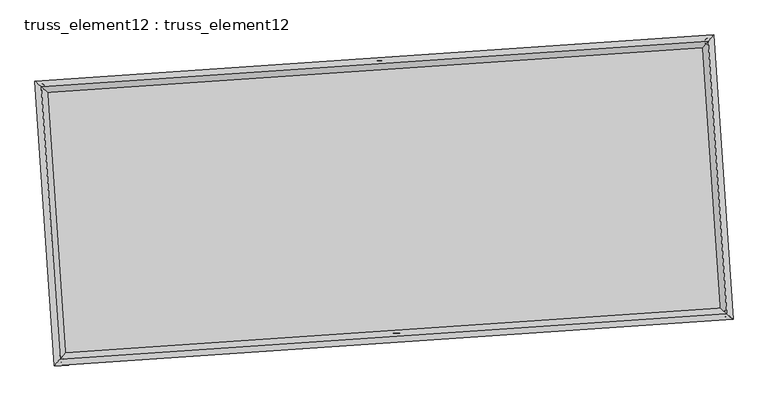
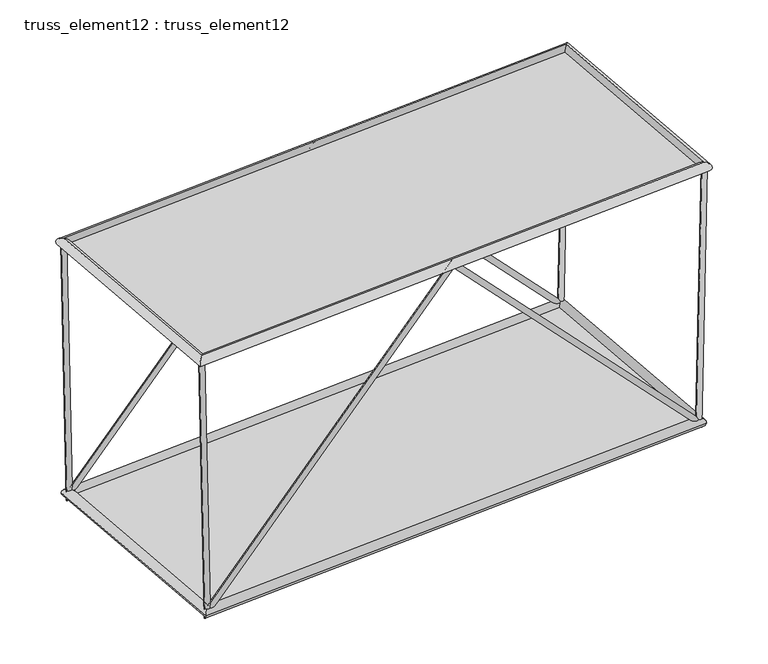
"""IFC4 building model written with IfcOpenShell, lengths in millimetres: plate geometry, truss_element12 : truss_element12."""

import ifcopenshell
import ifcopenshell.guid

model = None  # the IFC model being written
_history = None  # IfcOwnerHistory: only IFC2X3 demands one
_inside = {}  # id of a spatial element -> (the spatial element, [elements in it])
_under = {}  # id of a project, library or spatial element -> (it, [spatial elements below it])
_declared = {}  # id of a project -> (the project, [libraries it declares])
_typed = {}  # id of a type object -> (the type object, [elements of that type])
_made_of = {}  # id of a material, layer set ... -> (it, [elements and type objects made of it])


def new_model(schema):
    """Start an empty IFC model of exactly this schema.

    Asked for "IFC4X3", IfcOpenShell would pick the latest addendum, in which some entities
    have other attributes; the version numbers below select the first issue.
    IFC2X3 requires an IfcOwnerHistory on every rooted entity: one is made here for all.
    """
    global model, _history
    if schema == "IFC4X3":
        model = ifcopenshell.file(schema_version=(4, 3, 0, 0))
    else:
        model = ifcopenshell.file(schema=schema)
    _inside.clear()
    _under.clear()
    _declared.clear()
    _typed.clear()
    _made_of.clear()
    _history = None
    if model.schema == "IFC2X3":
        org = make("IfcOrganization", Name="unknown")
        user = make(
            "IfcPersonAndOrganization",
            ThePerson=make("IfcPerson", FamilyName="unknown"),
            TheOrganization=org,
        )
        app = make(
            "IfcApplication",
            ApplicationDeveloper=org,
            Version="unknown",
            ApplicationFullName="unknown",
            ApplicationIdentifier="unknown",
        )
        _history = make(
            "IfcOwnerHistory",
            OwningUser=user,
            OwningApplication=app,
            ChangeAction="ADDED",
            CreationDate=0,
        )
    return model


def make(cls, **values):
    """One entity of the class cls with the attributes given. An attribute that is None is left unset."""
    return model.create_entity(
        cls, **{name: value for name, value in values.items() if value is not None}
    )


def rooted(cls, **values):
    """An entity with a GlobalId (a new one), such as an element, a storey or a relation."""
    return make(cls, GlobalId=ifcopenshell.guid.new(), OwnerHistory=_history, **values)


def si_unit(unit_type, name, prefix=None):
    """IfcSIUnit, for example si_unit("LENGTHUNIT", "METRE", prefix="MILLI")."""
    return make("IfcSIUnit", UnitType=unit_type, Prefix=prefix, Name=name)


def assignment(units):
    """IfcUnitAssignment: the units of a project."""
    return None if units is None else make("IfcUnitAssignment", Units=units)


def point(xyz):
    """IfcCartesianPoint."""
    return None if xyz is None else make("IfcCartesianPoint", Coordinates=xyz)


def direction(xyz):
    """IfcDirection."""
    return None if xyz is None else make("IfcDirection", DirectionRatios=xyz)


def frame(location, z_axis=None, x_axis=None):
    """IfcAxis2Placement3D, a coordinate frame: its origin and axes. An axis left out is left unset."""
    return make(
        "IfcAxis2Placement3D",
        Location=point(location),
        Axis=direction(z_axis),
        RefDirection=direction(x_axis),
    )


def origin():
    """The frame at (0, 0, 0) with its axes left unset."""
    return frame((0.0, 0.0, 0.0))


def origin_with_axes():
    """The frame at (0, 0, 0) with the z axis (0, 0, 1) and the x axis (1, 0, 0) written out."""
    return frame((0.0, 0.0, 0.0), z_axis=(0.0, 0.0, 1.0), x_axis=(1.0, 0.0, 0.0))


def place(relative_to, where):
    """IfcLocalPlacement: puts the frame where relative to a parent placement (None: the world)."""
    return make(
        "IfcLocalPlacement", PlacementRelTo=relative_to, RelativePlacement=where
    )


def context(
    kind, dimensions, precision=None, world=None, true_north=None, identifier=None
):
    """IfcGeometricRepresentationContext, for example the 3D "Model" context."""
    return make(
        "IfcGeometricRepresentationContext",
        ContextIdentifier=identifier,
        ContextType=kind,
        CoordinateSpaceDimension=dimensions,
        Precision=precision,
        WorldCoordinateSystem=world,
        TrueNorth=true_north,
    )


def project(units=None, contexts=None):
    """IfcProject with its units and contexts."""
    return rooted(
        "IfcProject",
        Name="project",
        RepresentationContexts=contexts,
        UnitsInContext=assignment(units),
    )


def spatial(cls, under=None, at=None, **own):
    """A site, building, storey or space (cls), placed at a placement, below another one or the project."""
    s = rooted(cls, ObjectPlacement=at, **own)
    if under is not None:
        _under.setdefault(under.id(), (under, []))[1].append(s)
    return s


def polyline(points):
    """IfcPolyline through the points."""
    return make("IfcPolyline", Points=[point(p) for p in points])


def circle_curve(where, radius):
    """IfcCircle in the frame where."""
    return make("IfcCircle", Position=where, Radius=radius)


def ellipse_curve(where, semi_axis1, semi_axis2):
    """IfcEllipse in the frame where."""
    return make(
        "IfcEllipse", Position=where, SemiAxis1=semi_axis1, SemiAxis2=semi_axis2
    )


def outline(outer, holes=None, kind="AREA"):
    """IfcArbitraryClosedProfileDef: a profile drawn as a closed curve; with holes, ...WithVoids."""
    if holes is None:
        return make("IfcArbitraryClosedProfileDef", ProfileType=kind, OuterCurve=outer)
    return make(
        "IfcArbitraryProfileDefWithVoids",
        ProfileType=kind,
        OuterCurve=outer,
        InnerCurves=holes,
    )


def extrude(swept, where, along, depth):
    """IfcExtrudedAreaSolid: the profile swept, set in the frame where, extruded along a direction by depth."""
    return make(
        "IfcExtrudedAreaSolid",
        SweptArea=swept,
        Position=where,
        ExtrudedDirection=direction(along),
        Depth=depth,
    )


def shape(context_of_items, identifier, shape_type, items):
    """IfcShapeRepresentation: the items that make up one representation, for example the "Body"."""
    return make(
        "IfcShapeRepresentation",
        ContextOfItems=context_of_items,
        RepresentationIdentifier=identifier,
        RepresentationType=shape_type,
        Items=items,
    )


def source(mapping_origin, context_of_items, identifier, shape_type, items):
    """IfcRepresentationMap: a shape defined once, which mapped items show again and again."""
    return make(
        "IfcRepresentationMap",
        MappingOrigin=mapping_origin,
        MappedRepresentation=shape(context_of_items, identifier, shape_type, items),
    )


def transform(
    local_origin,
    x_axis=None,
    y_axis=None,
    z_axis=None,
    scale=None,
    scale2=None,
    scale3=None,
    uniform=True,
):
    """IfcCartesianTransformationOperator3D, or its non-uniform kind. x_axis, y_axis, z_axis: its Axis1, 2, 3."""
    if uniform:
        return make(
            "IfcCartesianTransformationOperator3D",
            Axis1=direction(x_axis),
            Axis2=direction(y_axis),
            LocalOrigin=point(local_origin),
            Scale=scale,
            Axis3=direction(z_axis),
        )
    return make(
        "IfcCartesianTransformationOperator3DnonUniform",
        Axis1=direction(x_axis),
        Axis2=direction(y_axis),
        LocalOrigin=point(local_origin),
        Scale=scale,
        Axis3=direction(z_axis),
        Scale2=scale2,
        Scale3=scale3,
    )


def mapped(mapping_source, mapping_target):
    """IfcMappedItem: shows the shape of a source again, moved by a transform."""
    return make(
        "IfcMappedItem", MappingSource=mapping_source, MappingTarget=mapping_target
    )


def made_of(thing, what):
    """Note that an element or type object is made of a material, layer set ...; save() writes the relation."""
    if what is not None:
        _made_of.setdefault(what.id(), (what, []))[1].append(thing)
    return thing


def element(
    cls,
    number,
    at=None,
    inside=None,
    cuts=None,
    type_object=None,
    material=None,
    context=None,
    identifier="Body",
    shape_type=None,
    held_by="IfcProductDefinitionShape",
    body=None,
    shapes=None,
    **own,
):
    """One element of the class cls, such as IfcWall. Its Tag is "e" and its number.

    at: its placement. inside: the storey or other place that contains it. cuts: it is an
    opening in that element (IfcRelVoidsElement). A single representation is given by context,
    identifier, shape_type and body (its items); several are given by shapes. held_by: the class
    of the entity that holds the representations. save() writes the other relations.
    """
    e = rooted(cls, Tag="e%d" % number, ObjectPlacement=at, **own)
    if body is not None:
        shapes = [shape(context, identifier, shape_type, body)]
    if shapes is not None:
        e.Representation = make(held_by, Representations=shapes)
    if inside is not None:
        _inside.setdefault(inside.id(), (inside, []))[1].append(e)
    if cuts is not None:
        rooted(
            "IfcRelVoidsElement", RelatingBuildingElement=cuts, RelatedOpeningElement=e
        )
    if type_object is not None:
        _typed.setdefault(type_object.id(), (type_object, []))[1].append(e)
    return made_of(e, material)


def aggregate(whole, parts):
    """IfcRelAggregates: a whole, such as a stair, and the parts it consists of."""
    return rooted("IfcRelAggregates", RelatingObject=whole, RelatedObjects=parts)


def save(model, path):
    """Write the relations noted so far, then the file.

    IfcRelAggregates (storeys below a building ...), IfcRelContainedInSpatialStructure (elements
    in a storey), IfcRelDefinesByType, IfcRelAssociatesMaterial and IfcRelDeclares: one each for
    every whole, place, type object, material and project.
    """
    for whole, parts in _under.values():
        aggregate(whole, parts)
    for where, things in _inside.values():
        rooted(
            "IfcRelContainedInSpatialStructure",
            RelatedElements=things,
            RelatingStructure=where,
        )
    for kind, things in _typed.values():
        rooted("IfcRelDefinesByType", RelatedObjects=things, RelatingType=kind)
    for what, things in _made_of.values():
        rooted("IfcRelAssociatesMaterial", RelatedObjects=things, RelatingMaterial=what)
    for by, libraries in _declared.values():
        rooted("IfcRelDeclares", RelatingContext=by, RelatedDefinitions=libraries)
    model.write(path)


def plane_surface(at):
    """IfcPlane: the flat surface through the origin of the frame at, square to its z axis."""
    return make("IfcPlane", Position=at)


def cylinder_surface(at, radius):
    """IfcCylindricalSurface: all points at the distance radius from the z axis of the frame at."""
    return make("IfcCylindricalSurface", Position=at, Radius=radius)


def advanced_brep(points, edges, surfaces, faces):
    """IfcAdvancedBrep: a solid bounded by faces that lie on surfaces and meet in shared edges.

    An edge is (start, end): straight between two places in points (the first is 0);
    or (start, end, curve); or (start, end, curve, False) where it runs against its curve.
    A face is (place in surfaces, loops), or (place, loops, False) where it looks against
    its surface's normal. A loop lists edges by number (the first is 1), with a minus sign
    where the edge is run from its end to its start. The first loop is the outer one.
    """
    corners = [point(p) for p in points]
    vertices = [make("IfcVertexPoint", VertexGeometry=c) for c in corners]
    made = []
    for start, end, *more in edges:
        made.append(
            make(
                "IfcEdgeCurve",
                EdgeStart=vertices[start],
                EdgeEnd=vertices[end],
                EdgeGeometry=more[0] if more else make("IfcPolyline", Points=[corners[start], corners[end]]),
                SameSense=more[1] if len(more) > 1 else True,
            )
        )
    hull = []
    for where, loops, *sense in faces:
        bounds = []
        for j, loop in enumerate(loops):
            ring = [make("IfcOrientedEdge", EdgeElement=made[abs(k) - 1], Orientation=k > 0) for k in loop]
            bounds.append(
                make(
                    "IfcFaceOuterBound" if j == 0 else "IfcFaceBound",
                    Bound=make("IfcEdgeLoop", EdgeList=ring),
                    Orientation=True,
                )
            )
        hull.append(make("IfcAdvancedFace", Bounds=bounds, FaceSurface=surfaces[where], SameSense=sense[0] if sense else True))
    return make("IfcAdvancedBrep", Outer=make("IfcClosedShell", CfsFaces=hull))


def truss_element12_truss_element12_abe7b1e7(model_context):
    return source(origin(), model_context, "Body", "SolidModel", [
        advanced_brep(
        [(-3770.8878019, 2268.9998903, 4999.9319376), (-3869.9687215, 2255.6402044, 4997.8129357), (-3667.5052192, 2276.0491556, 121.4949725), (-3761.4816636, 2263.0375245, -121.4949725), (1064.3047665, 2598.6932913, 5070.9753827), (1064.7442266, 2592.1195217, 4926.7446167), (5794.9719015, 2921.2595003, 121.4870027), (5889.7890755, 2921.1209882, -121.4870027), (5899.4888428, 2928.3861132, 4999.9186849), (5999.4656666, 2928.5994181, 4997.7764407)],
        [
            (0, 1, circle_curve(frame((-3820.4282617, 2262.3200473, 4998.8724366), z_axis=(-0.021186964059823055, -0.0014446585400489402, 0.9997744873298331), x_axis=(-0.1335973438749746, 0.9910347078393886, -0.0013991308907449146)), 50.0)),
            (1, 0, circle_curve(frame((-3820.4282617, 2262.3200473, 4998.8724366), z_axis=(-0.021186964059823055, -0.0014446585400489402, 0.9997744873298331), x_axis=(-0.1335973438749746, 0.9910347078393886, -0.0013991308907449146)), 50.0)),
            (0, 2),
            (2, 3, ellipse_curve(frame((-3714.4934414, 2269.54334, 0.0), z_axis=(-0.9296544314303254, -0.06338960173189395, 0.36293855749180226), x_axis=(0.36209777260493814, 0.02469007065143342, 0.9318130732533052)), 130.6694735, 50.0)),
            (3, 1),
            (3, 2, ellipse_curve(frame((-3714.4934414, 2269.54334, 0.0), z_axis=(-0.9296544314303254, -0.06338960173189395, 0.36293855749180226), x_axis=(0.36209777260493814, 0.02469007065143342, 0.9318130732533052)), 130.6694735, 50.0)),
            (2, 4),
            (4, 5, ellipse_curve(frame((1064.5244965, 2595.4064065, 4998.8599997), z_axis=(-0.9976833942347468, -0.06802823810322978, 6.073553142189921e-05), x_axis=(-6.0594831251560616e-05, -4.131731200348947e-06, -0.9999999981555977)), 72.2724119, 50.0)),
            (5, 3),
            (5, 4, ellipse_curve(frame((1064.5244965, 2595.4064065, 4998.8599997), z_axis=(-0.9976833942347468, -0.06802823810322978, 6.073553142189921e-05), x_axis=(-6.0594831251560616e-05, -4.131731200348947e-06, -0.9999999981555977)), 72.2724119, 50.0)),
            (4, 6),
            (6, 7, ellipse_curve(frame((5842.3804885, 2921.1902443, 0.0), z_axis=(-0.929718590145964, -0.06339397647082363, -0.3627734098362472), x_axis=(-0.36193300753109015, -0.024678835947378536, 0.9318773809443935)), 130.6518852, 50.0)),
            (7, 5),
            (7, 6, ellipse_curve(frame((5842.3804885, 2921.1902443, 0.0), z_axis=(-0.929718590145964, -0.06339397647082363, -0.3627734098362472), x_axis=(-0.36193300753109015, -0.024678835947378536, 0.9318773809443935)), 130.6518852, 50.0)),
            (8, 9, circle_curve(frame((5949.4772547, 2928.4927656, 4998.8475628), z_axis=(0.021419353246380234, 0.001460504275286309, 0.9997695125546532), x_axis=(-0.0021638448984886293, 0.999996658509091, -0.0014144772560226867)), 50.0)),
            (9, 8, circle_curve(frame((5949.4772547, 2928.4927656, 4998.8475628), z_axis=(0.021419353246380234, 0.001460504275286309, 0.9997695125546532), x_axis=(-0.0021638448984886293, 0.999996658509091, -0.0014144772560226867)), 50.0)),
            (6, 8),
            (9, 7),
        ],
        [
            plane_surface(frame((-3820.4282617, 2312.3199951, 4998.9446858), z_axis=(-0.021186964059822382, -0.0014446585400488944, 0.9997744873298331), x_axis=(0.9997755310838168, -3.061480063770717e-05, 0.021186941940879226))),
            cylinder_surface(frame((-3820.4282617, 2262.3200473, 4998.8724366), z_axis=(-0.021186964059823055, -0.0014446585400489402, 0.9997744873298331), x_axis=(-0.1335973438749746, 0.9910347078393886, -0.0013991308907449146)), 50.0),
            cylinder_surface(frame((-3714.4934414, 2269.54334, 0.0), z_axis=(-0.6902679812639986, -0.047066749688142194, -0.7220213536423408), x_axis=(-0.02042071364567827, 0.9987517920300755, -0.045583465981802296)), 50.0),
            cylinder_surface(frame((1064.5244965, 2595.4064065, 4998.8599997), z_axis=(-0.6901804746474645, -0.0470607829446048, 0.7221053905933964), x_axis=(-0.11534567202188306, 0.9922792199619508, -0.045577687277029266)), 50.0),
            plane_surface(frame((5949.4772547, 2878.492819, 4998.9206047), z_axis=(0.02141935324638098, 0.0014605042752824204, 0.9997695125546532), x_axis=(0.999770579336333, -3.129023561676551e-05, -0.021419330391363928))),
            cylinder_surface(frame((5842.3804885, 2921.1902443, 0.0), z_axis=(-0.021419353246380234, -0.001460504275286309, -0.9997695125546532), x_axis=(-0.0021638448984886293, 0.999996658509091, -0.0014144772560226867)), 50.0),
        ],
        [
            (0, [[1, 2]]),
            (1, [[-1, 3, 4, 5]]),
            (1, [[-2, -5, 6, -3]]),
            (2, [[-4, 7, 8, 9]]),
            (2, [[-6, -9, 10, -7]]),
            (3, [[-8, 11, 12, 13]]),
            (3, [[-10, -13, 14, -11]]),
            (4, [[15, 16]]),
            (5, [[-12, 17, -16, 18]]),
            (5, [[-14, -18, -15, -17]]),
        ],
    ),
        advanced_brep(
        [(-3498.774849, -1721.733694, 4999.9319376), (-3597.8557686, -1735.0933799, 4997.8129357), (-3395.3922663, -1714.6844287, 121.4949725), (-3489.3687107, -1727.6960598, -121.4949725), (1336.4177194, -1392.040293, 5070.9753827), (1336.8571795, -1398.6140626, 4926.7446167), (6067.0848544, -1069.474084, 121.4870027), (6161.9020284, -1069.6125961, -121.4870027), (6171.6017958, -1062.3474711, 4999.9186849), (6271.5786195, -1062.1341662, 4997.7764407)],
        [
            (0, 1, circle_curve(frame((-3548.3153088, -1728.413537, 4998.8724366), z_axis=(-0.021186964059823104, -0.001444658540048999, 0.9997744873298331), x_axis=(-0.13359734387497507, 0.9910347078393886, -0.0013991308907448728)), 50.0)),
            (1, 0, circle_curve(frame((-3548.3153088, -1728.413537, 4998.8724366), z_axis=(-0.021186964059823104, -0.001444658540048999, 0.9997744873298331), x_axis=(-0.13359734387497507, 0.9910347078393886, -0.0013991308907448728)), 50.0)),
            (0, 2),
            (2, 3, ellipse_curve(frame((-3442.3804885, -1721.1902443, 0.0), z_axis=(-0.9296544314303253, -0.06338960173189416, 0.36293855749180204), x_axis=(0.3620977726049378, 0.02469007065143343, 0.9318130732533053)), 130.6694735, 50.0)),
            (3, 1),
            (3, 2, ellipse_curve(frame((-3442.3804885, -1721.1902443, 0.0), z_axis=(-0.9296544314303253, -0.06338960173189416, 0.36293855749180204), x_axis=(0.3620977726049378, 0.02469007065143343, 0.9318130732533053)), 130.6694735, 50.0)),
            (2, 4),
            (4, 5, ellipse_curve(frame((1336.6374494, -1395.3271778, 4998.8599997), z_axis=(-0.9976833942347471, -0.06802823810322975, 6.073553142173877e-05), x_axis=(-6.059483125109933e-05, -4.1317312005027025e-06, -0.9999999981555977)), 72.2724119, 50.0)),
            (5, 3),
            (5, 4, ellipse_curve(frame((1336.6374494, -1395.3271778, 4998.8599997), z_axis=(-0.9976833942347471, -0.06802823810322975, 6.073553142173877e-05), x_axis=(-6.059483125109933e-05, -4.1317312005027025e-06, -0.9999999981555977)), 72.2724119, 50.0)),
            (4, 6),
            (6, 7, ellipse_curve(frame((6114.4934414, -1069.54334, 0.0), z_axis=(-0.929718590145964, -0.06339397647082334, -0.3627734098362472), x_axis=(-0.36193300753109015, -0.024678835947378446, 0.9318773809443935)), 130.6518852, 50.0)),
            (7, 5),
            (7, 6, ellipse_curve(frame((6114.4934414, -1069.54334, 0.0), z_axis=(-0.929718590145964, -0.06339397647082334, -0.3627734098362472), x_axis=(-0.36193300753109015, -0.024678835947378446, 0.9318773809443935)), 130.6518852, 50.0)),
            (8, 9, circle_curve(frame((6221.5902076, -1062.2408187, 4998.8475628), z_axis=(0.021419353246380123, 0.0014605042752862665, 0.9997695125546532), x_axis=(-0.0021638448984882684, 0.999996658509091, -0.001414477256022652)), 50.0)),
            (9, 8, circle_curve(frame((6221.5902076, -1062.2408187, 4998.8475628), z_axis=(0.021419353246380123, 0.0014605042752862665, 0.9997695125546532), x_axis=(-0.0021638448984882684, 0.999996658509091, -0.001414477256022652)), 50.0)),
            (6, 8),
            (9, 7),
        ],
        [
            plane_surface(frame((-3548.3153088, -1678.4135892, 4998.9446858), z_axis=(-0.021186964059822382, -0.001444658540048914, 0.9997744873298331), x_axis=(0.9997755310838168, -3.061480063770717e-05, 0.021186941940879226))),
            cylinder_surface(frame((-3548.3153088, -1728.413537, 4998.8724366), z_axis=(-0.021186964059823104, -0.001444658540048999, 0.9997744873298331), x_axis=(-0.13359734387497507, 0.9910347078393886, -0.0013991308907448728)), 50.0),
            cylinder_surface(frame((-3442.3804885, -1721.1902443, 0.0), z_axis=(-0.6902679812639982, -0.04706674968814228, -0.722021353642341), x_axis=(-0.020420713645678303, 0.9987517920300755, -0.04558346598180237)), 50.0),
            cylinder_surface(frame((1336.6374494, -1395.3271778, 4998.8599997), z_axis=(-0.6901804746474646, -0.04706078294460461, 0.7221053905933964), x_axis=(-0.11534567202188295, 0.9922792199619508, -0.04557768727702941)), 50.0),
            plane_surface(frame((6221.5902076, -1112.2407653, 4998.9206047), z_axis=(0.021419353246380984, 0.0014605042752824403, 0.9997695125546533), x_axis=(0.999770579336333, -3.129023561676551e-05, -0.021419330391363928))),
            cylinder_surface(frame((6114.4934414, -1069.54334, 0.0), z_axis=(-0.021419353246380123, -0.0014605042752862665, -0.9997695125546532), x_axis=(-0.0021638448984882684, 0.999996658509091, -0.001414477256022652)), 50.0),
        ],
        [
            (0, [[1, 2]]),
            (1, [[-1, 3, 4, 5]]),
            (1, [[-2, -5, 6, -3]]),
            (2, [[-4, 7, 8, 9]]),
            (2, [[-6, -9, 10, -7]]),
            (3, [[-8, 11, 12, 13]]),
            (3, [[-10, -13, 14, -11]]),
            (4, [[15, 16]]),
            (5, [[-12, 17, -16, 18]]),
            (5, [[-14, -18, -15, -17]]),
        ],
    ),
        advanced_brep(
        [(-3548.3217778, -1728.4207068, 4908.8724369), (-3548.3088398, -1728.4063671, 5088.8724364), (-3820.4208794, 2262.313822, 5088.8724364), (-3820.4356441, 2262.3262727, 4908.8724369), (5949.4712419, 2928.4856269, 5088.8475625), (5949.4832676, 2928.4999043, 4908.847563), (6221.5832815, -1062.2345622, 5088.8475625), (6221.5971338, -1062.2470751, 4908.847563)],
        [
            (0, 1, ellipse_curve(frame((-3548.3153088, -1728.413537, 4998.8724366), z_axis=(-0.7535719234031808, 0.6573654662782376, 1.7961013785977973e-06), x_axis=(-0.6573654662758065, -0.7535719234053014, 1.7961013785979447e-06)), 127.2792206, 90.0)),
            (1, 2),
            (2, 3, ellipse_curve(frame((-3820.4282617, 2262.3200473, 4998.8724366), z_axis=(-0.6573654662758065, -0.7535719234053015, 1.796101378598083e-06), x_axis=(0.7535719234031809, -0.6573654662782374, -1.796101378597936e-06)), 127.2792206, 90.0)),
            (3, 0),
            (1, 0, ellipse_curve(frame((-3548.3153088, -1728.413537, 4998.8724366), z_axis=(-0.7535719234031808, 0.6573654662782376, 1.7961013785977973e-06), x_axis=(-0.6573654662758065, -0.7535719234053014, 1.7961013785979447e-06)), 127.2792206, 90.0)),
            (3, 2, ellipse_curve(frame((-3820.4282617, 2262.3200473, 4998.8724366), z_axis=(-0.6573654662758065, -0.7535719234053015, 1.796101378598083e-06), x_axis=(0.7535719234031809, -0.6573654662782374, -1.796101378597936e-06)), 127.2792206, 90.0)),
            (2, 4),
            (4, 5, ellipse_curve(frame((5949.4772547, 2928.4927656, 4998.8475628), z_axis=(-0.7535719234031808, 0.6573654662782376, 1.7961013785980747e-06), x_axis=(-0.6573654662758065, -0.7535719234053013, 1.796101378597944e-06)), 127.2792206, 90.0)),
            (5, 3),
            (5, 4, ellipse_curve(frame((5949.4772547, 2928.4927656, 4998.8475628), z_axis=(-0.7535719234031808, 0.6573654662782376, 1.7961013785980747e-06), x_axis=(-0.6573654662758065, -0.7535719234053013, 1.796101378597944e-06)), 127.2792206, 90.0)),
            (4, 6),
            (6, 7, ellipse_curve(frame((6221.5902076, -1062.2408187, 4998.8475628), z_axis=(0.6573654662758065, 0.7535719234053013, -1.7961013785978055e-06), x_axis=(-0.7535719234031807, 0.6573654662782378, 1.796101378597936e-06)), 127.2792206, 90.0)),
            (7, 5),
            (7, 6, ellipse_curve(frame((6221.5902076, -1062.2408187, 4998.8475628), z_axis=(0.6573654662758065, 0.7535719234053013, -1.7961013785978055e-06), x_axis=(-0.7535719234031807, 0.6573654662782378, 1.796101378597936e-06)), 127.2792206, 90.0)),
            (6, 1),
            (0, 7),
        ],
        [
            cylinder_surface(frame((-3548.3153088, -1728.413537, 4998.8724366), z_axis=(0.06802823822869959, -0.9976833960748769, 0.0), x_axis=(-0.9976833931072083, -0.06802823802634556, 7.713052989592242e-05)), 90.0),
            cylinder_surface(frame((-3820.4282617, 2262.3200473, 4998.8724366), z_axis=(-0.9976833960716583, -0.06802823822847938, 2.540070929010318e-06), x_axis=(-0.0680282378504271, 0.997683393312342, 7.459045897397833e-05)), 90.0),
            cylinder_surface(frame((5949.4772547, 2928.4927656, 4998.8475628), z_axis=(-0.06802823822869955, 0.997683396074877, 0.0), x_axis=(0.9976833934852606, 0.06802823805212346, 7.205038805203428e-05)), 90.0),
            cylinder_surface(frame((6221.5902076, -1062.2408187, 4998.8475628), z_axis=(0.9976833960716583, 0.06802823822847945, -2.5400709290101224e-06), x_axis=(0.06802823822847945, -0.997683393286564, 7.459045897397836e-05)), 90.0),
        ],
        [
            (0, [[1, 2, 3, 4]]),
            (0, [[5, -4, 6, -2]]),
            (1, [[-3, 7, 8, 9]]),
            (1, [[-6, -9, 10, -7]]),
            (2, [[-8, 11, 12, 13]]),
            (2, [[-10, -13, 14, -11]]),
            (3, [[-12, 15, -1, 16]]),
            (3, [[-14, -16, -5, -15]]),
        ],
    ),
        advanced_brep(
        [(-3358.7115243, -1625.2761972, 0.0), (-3526.0494527, -1817.1042913, 0.0), (-3810.4074885, 2353.2123043, 0.0), (-3618.5793943, 2185.8743758, 0.0), (5926.0494527, 3017.1042913, 0.0), (5758.7115243, 2825.2761972, 0.0), (6210.4074885, -1153.2123043, 0.0), (6018.5793943, -985.8743758, 0.0)],
        [
            (0, 1, ellipse_curve(frame((-3442.3804885, -1721.1902443, 0.0), z_axis=(-0.7535719234054581, 0.6573654662780808, 0.0), x_axis=(-0.6573654662780808, -0.7535719234054579, 0.0)), 127.2792206, 90.0)),
            (1, 2),
            (2, 3, ellipse_curve(frame((-3714.4934414, 2269.54334, 0.0), z_axis=(-0.6573654662780808, -0.753571923405458, 0.0), x_axis=(0.7535719234054581, -0.6573654662780807, 0.0)), 127.2792206, 90.0)),
            (3, 0),
            (1, 0, ellipse_curve(frame((-3442.3804885, -1721.1902443, 0.0), z_axis=(-0.7535719234054581, 0.6573654662780808, 0.0), x_axis=(-0.6573654662780808, -0.7535719234054579, 0.0)), 127.2792206, 90.0)),
            (3, 2, ellipse_curve(frame((-3714.4934414, 2269.54334, 0.0), z_axis=(-0.6573654662780808, -0.753571923405458, 0.0), x_axis=(0.7535719234054581, -0.6573654662780807, 0.0)), 127.2792206, 90.0)),
            (2, 4),
            (4, 5, ellipse_curve(frame((5842.3804885, 2921.1902443, 0.0), z_axis=(-0.7535719234054581, 0.6573654662780808, 0.0), x_axis=(-0.6573654662780806, -0.7535719234054581, 0.0)), 127.2792206, 90.0)),
            (5, 3),
            (5, 4, ellipse_curve(frame((5842.3804885, 2921.1902443, 0.0), z_axis=(-0.7535719234054581, 0.6573654662780808, 0.0), x_axis=(-0.6573654662780806, -0.7535719234054581, 0.0)), 127.2792206, 90.0)),
            (4, 6),
            (6, 7, ellipse_curve(frame((6114.4934414, -1069.54334, 0.0), z_axis=(0.6573654662780808, 0.753571923405458, 0.0), x_axis=(-0.753571923405458, 0.6573654662780808, 0.0)), 127.2792206, 90.0)),
            (7, 5),
            (7, 6, ellipse_curve(frame((6114.4934414, -1069.54334, 0.0), z_axis=(0.6573654662780808, 0.753571923405458, 0.0), x_axis=(-0.753571923405458, 0.6573654662780808, 0.0)), 127.2792206, 90.0)),
            (6, 1),
            (0, 7),
        ],
        [
            cylinder_surface(frame((-3442.3804885, -1721.1902443, 0.0), z_axis=(0.0680282382287018, -0.9976833960748765, 0.0), x_axis=(-0.9976833960748765, -0.0680282382287018, 0.0)), 90.0),
            cylinder_surface(frame((-3714.4934414, 2269.54334, 0.0), z_axis=(-0.9976833960748765, -0.06802823822870102, 0.0), x_axis=(-0.06802823822870102, 0.9976833960748765, 0.0)), 90.0),
            cylinder_surface(frame((5842.3804885, 2921.1902443, 0.0), z_axis=(-0.06802823822870162, 0.9976833960748765, 0.0), x_axis=(0.9976833960748765, 0.06802823822870162, 0.0)), 90.0),
            cylinder_surface(frame((6114.4934414, -1069.54334, 0.0), z_axis=(0.9976833960748767, 0.06802823822870084, 0.0), x_axis=(0.06802823822870084, -0.9976833960748767, 0.0)), 90.0),
        ],
        [
            (0, [[1, 2, 3, 4]]),
            (0, [[5, -4, 6, -2]]),
            (1, [[-3, 7, 8, 9]]),
            (1, [[-6, -9, 10, -7]]),
            (2, [[-8, 11, 12, 13]]),
            (2, [[-10, -13, 14, -11]]),
            (3, [[-12, 15, -1, 16]]),
            (3, [[-14, -16, -5, -15]]),
        ],
    ),
        extrude(outline(polyline([(-3442.3804885, -1721.1902443), (-3714.4934414, 2269.54334), (5842.3804885, 2921.1902443), (6114.4934414, -1069.54334), (-3442.3804885, -1721.1902443)])), origin_with_axes(), (0.0, 0.0, 1.0), 20.0),
        extrude(outline(polyline([(-2000.0, 4896.2955357), (2000.0, 4896.2955357), (2000.0, -4896.2955356), (-2000.0, -4896.2955356), (-2000.0, 4896.2955357)])), frame((1200.580973, 600.0396143, 4998.8599997), z_axis=(2.534186590725984e-06, 1.7279655027650736e-07, 0.9999999999967741), x_axis=(-0.06802823822870187, 0.9976833960748765, 0.0)), (0.0, 0.0, 1.0), 20.0),
    ])


if __name__ == "__main__":
    model = new_model("IFC4")
    model_context = context("Model", 3, world=origin())
    ifc_project = project(units=[si_unit("LENGTHUNIT", "METRE", prefix="MILLI")], contexts=[model_context])
    site = spatial("IfcSite", under=ifc_project)
    building = spatial("IfcBuilding", under=site)
    placement = place(None, origin())
    truss_element12_truss_element12_shape = truss_element12_truss_element12_abe7b1e7(model_context)
    element("IfcPlate", 1, ObjectType="truss_element12 : truss_element12", at=placement, inside=building, context=model_context, shape_type="MappedRepresentation", body=[
        mapped(truss_element12_truss_element12_shape, transform((0.0, 0.0, 0.0), x_axis=(1.0, 0.0, 0.0), y_axis=(0.0, 1.0, 0.0), z_axis=(0.0, 0.0, 1.0))),
    ])
    save(model, "model.ifc")

# Revit data of these elements
# Type "truss_element12 : truss_element12"
#   steellbar1 = 90 mm
#   steelbar2 = 50 mm
#   offset1 = 5000 mm
#   M = Default Roof
# Element 1 (IfcPlate, "truss_element12 : truss_element12")
#   Materials on its faces: "Default Roof"
# Materials
#   "Default Roof": class "Miscellaneous", colour RGB 0 127 0, transparency 0, Comments = "Rendering appearance not upgraded Rendering appearance not upgraded ", Cost = 0
